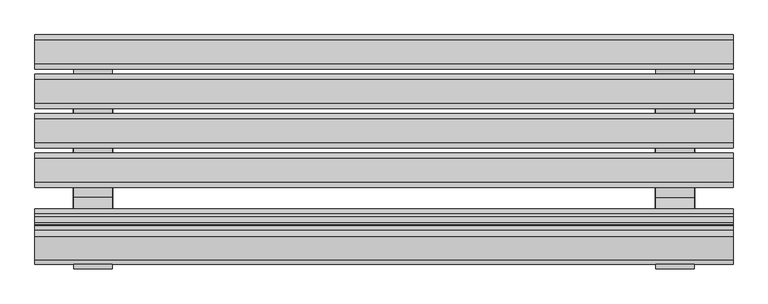
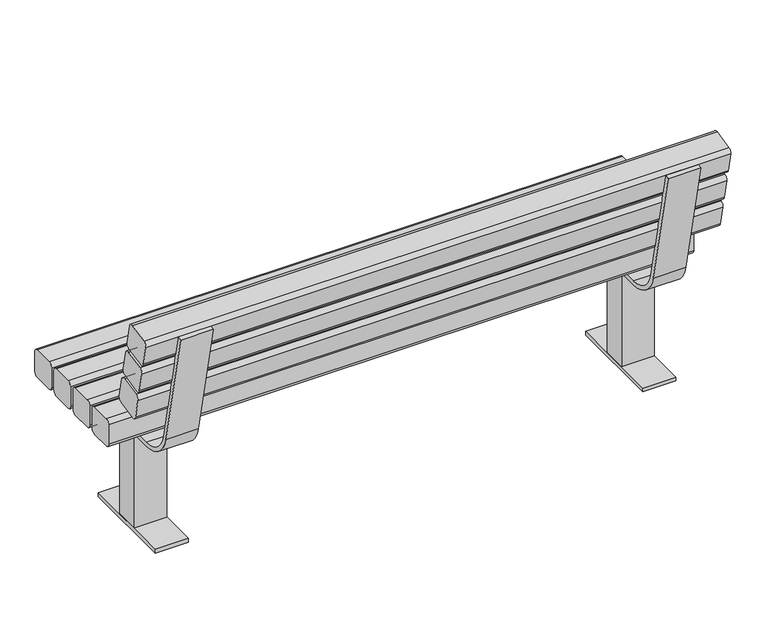
"""IFC4 building model written with IfcOpenShell, lengths in millimetres: furniture geometry, NLRS_90_FU_WPB_parkbank_gen_rsf : 1800mm breed."""

from ifc_helpers import new_model, si_unit, point, frame, frame_2d, origin, origin_with_axes, place, context, project, spatial, polyline, circle_curve, trimmed, segment, composite_curve, outline, extrude, source, transform, mapped, element, save


def furniture_d88922e8(model_context):
    return source(origin(), model_context, "Body", "SweptSolid", [
        extrude(outline(polyline([(-778.4316018, 207.3631555), (-778.4316018, 512.1631555), (-676.8316018, 512.1631555), (-676.8316018, 207.3631555), (-778.4316018, 207.3631555)])), origin_with_axes(), (0.0, 0.0, 1.0), 12.7),
        extrude(outline(polyline([(722.3683982, 321.6631555), (722.3683982, 397.8631555), (822.3683982, 397.8631555), (822.3683982, 321.6631555), (722.3683982, 321.6631555)])), frame((0.0, 0.0, 12.7), z_axis=(0.0, 0.0, 1.0), x_axis=(1.0, 0.0, 0.0)), (0.0, 0.0, 1.0), 304.8),
        extrude(outline(composite_curve([segment(polyline([(85.9429731, 777.6296037), (165.0207138, 405.5980841)]), True, "CONTINUOUS"), segment(trimmed(circle_curve(frame_2d((258.1892727, 425.4016727)), 95.25), [point((165.0207138, 405.5980841))], [point((258.1892727, 330.1516727))], True, "CARTESIAN"), True, "CONTINUOUS"), segment(polyline([(258.1892727, 330.1516727), (656.6612098, 330.1516727), (656.6612098, 317.5), (258.1790004, 317.5)]), True, "CONTINUOUS"), segment(trimmed(circle_curve(frame_2d((258.1790004, 425.45)), 107.95), [point((258.1790004, 317.5))], [point((152.5879669, 403.005933))], False, "CARTESIAN"), True, "CONTINUOUS"), segment(polyline([(152.5879669, 403.005933), (73.5204986, 774.9891252), (85.9429731, 777.6296037)]), True, "CONTINUOUS")], self_intersect=False)), frame((722.3683982, 0.0, 0.0), z_axis=(1.0, 0.0, 0.0), x_axis=(0.0, 1.0, 0.0)), (0.0, 0.0, 1.0), 100.0),
        extrude(outline(polyline([(-677.6316018, 321.6631555), (-777.6316018, 321.6631555), (-777.6316018, 397.8631555), (-677.6316018, 397.8631555), (-677.6316018, 321.6631555)])), frame((0.0, 0.0, 12.7), z_axis=(0.0, 0.0, 1.0), x_axis=(1.0, 0.0, 0.0)), (0.0, 0.0, 1.0), 304.8),
        extrude(outline(polyline([(823.1683982, 207.3631555), (721.5683982, 207.3631555), (721.5683982, 512.1631555), (823.1683982, 512.1631555), (823.1683982, 207.3631555)])), origin_with_axes(), (0.0, 0.0, 1.0), 12.7),
        extrude(outline(composite_curve([segment(trimmed(circle_curve(frame_2d((202.7254759, 594.7128821)), 12.7), [point((200.0849974, 607.1353566))], [point((215.1479504, 597.3533605))], False, "CARTESIAN"), True, "CONTINUOUS"), segment(polyline([(215.1479504, 597.3533605), (228.3503428, 535.2409879)]), True, "CONTINUOUS"), segment(trimmed(circle_curve(frame_2d((215.9278683, 532.6005094)), 12.7), [point((228.3503428, 535.2409879))], [point((218.5683467, 520.1780349))], False, "CARTESIAN"), True, "CONTINUOUS"), segment(polyline([(218.5683467, 520.1780349), (156.4559741, 506.9756425)]), True, "CONTINUOUS"), segment(trimmed(circle_curve(frame_2d((153.8154956, 519.398117)), 12.7), [point((156.4559741, 506.9756425))], [point((141.3930211, 516.7576386))], False, "CARTESIAN"), True, "CONTINUOUS"), segment(polyline([(141.3930211, 516.7576386), (128.1906287, 578.8700112)]), True, "CONTINUOUS"), segment(trimmed(circle_curve(frame_2d((140.6131032, 581.5104897)), 12.7), [point((128.1906287, 578.8700112))], [point((137.9726248, 593.9329642))], False, "CARTESIAN"), True, "CONTINUOUS"), segment(polyline([(137.9726248, 593.9329642), (200.0849974, 607.1353566)]), True, "CONTINUOUS")], self_intersect=False)), frame((-877.6316018, 0.0, 0.0), z_axis=(1.0, 0.0, 0.0), x_axis=(0.0, 1.0, 0.0)), (0.0, 0.0, 1.0), 1800.0),
        extrude(outline(composite_curve([segment(trimmed(circle_curve(frame_2d((181.6016481, 694.0926783)), 12.7), [point((178.9611696, 706.5151528))], [point((194.0241226, 696.7331568))], False, "CARTESIAN"), True, "CONTINUOUS"), segment(polyline([(194.0241226, 696.7331568), (207.226515, 634.6207841)]), True, "CONTINUOUS"), segment(trimmed(circle_curve(frame_2d((194.8040405, 631.9803056)), 12.7), [point((207.226515, 634.6207841))], [point((197.4445189, 619.5578311))], False, "CARTESIAN"), True, "CONTINUOUS"), segment(polyline([(197.4445189, 619.5578311), (135.3321463, 606.3554388)]), True, "CONTINUOUS"), segment(trimmed(circle_curve(frame_2d((132.6916678, 618.7779133)), 12.7), [point((135.3321463, 606.3554388))], [point((120.2691933, 616.1374348))], False, "CARTESIAN"), True, "CONTINUOUS"), segment(polyline([(120.2691933, 616.1374348), (107.0668009, 678.2498075)]), True, "CONTINUOUS"), segment(trimmed(circle_curve(frame_2d((119.4892755, 680.8902859)), 12.7), [point((107.0668009, 678.2498075))], [point((116.848797, 693.3127605))], False, "CARTESIAN"), True, "CONTINUOUS"), segment(polyline([(116.848797, 693.3127605), (178.9611696, 706.5151528)]), True, "CONTINUOUS")], self_intersect=False)), frame((-877.6316018, 0.0, 0.0), z_axis=(1.0, 0.0, 0.0), x_axis=(0.0, 1.0, 0.0)), (0.0, 0.0, 1.0), 1800.0),
        extrude(outline(composite_curve([segment(polyline([(85.9429731, 777.6296037), (165.0207138, 405.5980841)]), True, "CONTINUOUS"), segment(trimmed(circle_curve(frame_2d((258.1892727, 425.4016727)), 95.25), [point((165.0207138, 405.5980841))], [point((258.1892727, 330.1516727))], True, "CARTESIAN"), True, "CONTINUOUS"), segment(polyline([(258.1892727, 330.1516727), (656.6612098, 330.1516727), (656.6612098, 317.5), (258.1790004, 317.5)]), True, "CONTINUOUS"), segment(trimmed(circle_curve(frame_2d((258.1790004, 425.45)), 107.95), [point((258.1790004, 317.5))], [point((152.5879669, 403.005933))], False, "CARTESIAN"), True, "CONTINUOUS"), segment(polyline([(152.5879669, 403.005933), (73.5204986, 774.9891252), (85.9429731, 777.6296037)]), True, "CONTINUOUS")], self_intersect=False)), frame((-777.6316018, 0.0, 0.0), z_axis=(1.0, 0.0, 0.0), x_axis=(0.0, 1.0, 0.0)), (0.0, 0.0, 1.0), 100.0),
        extrude(outline(composite_curve([segment(trimmed(circle_curve(frame_2d((160.4778203, 793.4724745)), 12.7), [point((157.8373418, 805.8949491))], [point((172.9002948, 796.112953))], False, "CARTESIAN"), True, "CONTINUOUS"), segment(polyline([(172.9002948, 796.112953), (186.1026872, 734.0005804)]), True, "CONTINUOUS"), segment(trimmed(circle_curve(frame_2d((173.6802127, 731.3601019)), 12.7), [point((186.1026872, 734.0005804))], [point((176.3206912, 718.9376274))], False, "CARTESIAN"), True, "CONTINUOUS"), segment(polyline([(176.3206912, 718.9376274), (114.2083185, 705.735235)]), True, "CONTINUOUS"), segment(trimmed(circle_curve(frame_2d((111.56784, 718.1577095)), 12.7), [point((114.2083185, 705.735235))], [point((99.1453655, 715.517231))], False, "CARTESIAN"), True, "CONTINUOUS"), segment(polyline([(99.1453655, 715.517231), (85.9429731, 777.6296037)]), True, "CONTINUOUS"), segment(trimmed(circle_curve(frame_2d((98.3654477, 780.2700822)), 12.7), [point((85.9429731, 777.6296037))], [point((95.7249692, 792.6925567))], False, "CARTESIAN"), True, "CONTINUOUS"), segment(polyline([(95.7249692, 792.6925567), (157.8373418, 805.8949491)]), True, "CONTINUOUS")], self_intersect=False)), frame((-877.6316018, 0.0, 0.0), z_axis=(1.0, 0.0, 0.0), x_axis=(0.0, 1.0, 0.0)), (0.0, 0.0, 1.0), 1800.0),
        extrude(outline(composite_curve([segment(trimmed(circle_curve(frame_2d((665.0298429, 406.3516727)), 12.7), [point((665.0298429, 419.0516727))], [point((677.7298429, 406.3516727))], False, "CARTESIAN"), True, "CONTINUOUS"), segment(polyline([(677.7298429, 406.3516727), (677.7298429, 342.8516727)]), True, "CONTINUOUS"), segment(trimmed(circle_curve(frame_2d((665.0298429, 342.8516727)), 12.7), [point((677.7298429, 342.8516727))], [point((665.0298429, 330.1516727))], False, "CARTESIAN"), True, "CONTINUOUS"), segment(polyline([(665.0298429, 330.1516727), (601.5298429, 330.1516727)]), True, "CONTINUOUS"), segment(trimmed(circle_curve(frame_2d((601.5298429, 342.8516727)), 12.7), [point((601.5298429, 330.1516727))], [point((588.8298429, 342.8516727))], False, "CARTESIAN"), True, "CONTINUOUS"), segment(polyline([(588.8298429, 342.8516727), (588.8298429, 406.3516727)]), True, "CONTINUOUS"), segment(trimmed(circle_curve(frame_2d((601.5298429, 406.3516727)), 12.7), [point((588.8298429, 406.3516727))], [point((601.5298429, 419.0516727))], False, "CARTESIAN"), True, "CONTINUOUS"), segment(polyline([(601.5298429, 419.0516727), (665.0298429, 419.0516727)]), True, "CONTINUOUS")], self_intersect=False)), frame((-877.6316018, 0.0, 0.0), z_axis=(1.0, 0.0, 0.0), x_axis=(0.0, 1.0, 0.0)), (0.0, 0.0, 1.0), 1800.0),
        extrude(outline(composite_curve([segment(trimmed(circle_curve(frame_2d((563.4298429, 406.3516727)), 12.7), [point((563.4298429, 419.0516727))], [point((576.1298429, 406.3516727))], False, "CARTESIAN"), True, "CONTINUOUS"), segment(polyline([(576.1298429, 406.3516727), (576.1298429, 342.8516727)]), True, "CONTINUOUS"), segment(trimmed(circle_curve(frame_2d((563.4298429, 342.8516727)), 12.7), [point((576.1298429, 342.8516727))], [point((563.4298429, 330.1516727))], False, "CARTESIAN"), True, "CONTINUOUS"), segment(polyline([(563.4298429, 330.1516727), (499.9298429, 330.1516727)]), True, "CONTINUOUS"), segment(trimmed(circle_curve(frame_2d((499.9298429, 342.8516727)), 12.7), [point((499.9298429, 330.1516727))], [point((487.2298429, 342.8516727))], False, "CARTESIAN"), True, "CONTINUOUS"), segment(polyline([(487.2298429, 342.8516727), (487.2298429, 406.3516727)]), True, "CONTINUOUS"), segment(trimmed(circle_curve(frame_2d((499.9298429, 406.3516727)), 12.7), [point((487.2298429, 406.3516727))], [point((499.9298429, 419.0516727))], False, "CARTESIAN"), True, "CONTINUOUS"), segment(polyline([(499.9298429, 419.0516727), (563.4298429, 419.0516727)]), True, "CONTINUOUS")], self_intersect=False)), frame((-877.6316018, 0.0, 0.0), z_axis=(1.0, 0.0, 0.0), x_axis=(0.0, 1.0, 0.0)), (0.0, 0.0, 1.0), 1800.0),
        extrude(outline(composite_curve([segment(trimmed(circle_curve(frame_2d((461.8298429, 406.3516727)), 12.7), [point((461.8298429, 419.0516727))], [point((474.5298429, 406.3516727))], False, "CARTESIAN"), True, "CONTINUOUS"), segment(polyline([(474.5298429, 406.3516727), (474.5298429, 342.8516727)]), True, "CONTINUOUS"), segment(trimmed(circle_curve(frame_2d((461.8298429, 342.8516727)), 12.7), [point((474.5298429, 342.8516727))], [point((461.8298429, 330.1516727))], False, "CARTESIAN"), True, "CONTINUOUS"), segment(polyline([(461.8298429, 330.1516727), (398.3298429, 330.1516727)]), True, "CONTINUOUS"), segment(trimmed(circle_curve(frame_2d((398.3298429, 342.8516727)), 12.7), [point((398.3298429, 330.1516727))], [point((385.6298429, 342.8516727))], False, "CARTESIAN"), True, "CONTINUOUS"), segment(polyline([(385.6298429, 342.8516727), (385.6298429, 406.3516727)]), True, "CONTINUOUS"), segment(trimmed(circle_curve(frame_2d((398.3298429, 406.3516727)), 12.7), [point((385.6298429, 406.3516727))], [point((398.3298429, 419.0516727))], False, "CARTESIAN"), True, "CONTINUOUS"), segment(polyline([(398.3298429, 419.0516727), (461.8298429, 419.0516727)]), True, "CONTINUOUS")], self_intersect=False)), frame((-877.6316018, 0.0, 0.0), z_axis=(1.0, 0.0, 0.0), x_axis=(0.0, 1.0, 0.0)), (0.0, 0.0, 1.0), 1800.0),
        extrude(outline(composite_curve([segment(trimmed(circle_curve(frame_2d((360.2298429, 406.3516727)), 12.7), [point((360.2298429, 419.0516727))], [point((372.9298429, 406.3516727))], False, "CARTESIAN"), True, "CONTINUOUS"), segment(polyline([(372.9298429, 406.3516727), (372.9298429, 342.8516727)]), True, "CONTINUOUS"), segment(trimmed(circle_curve(frame_2d((360.2298429, 342.8516727)), 12.7), [point((372.9298429, 342.8516727))], [point((360.2298429, 330.1516727))], False, "CARTESIAN"), True, "CONTINUOUS"), segment(polyline([(360.2298429, 330.1516727), (296.7298429, 330.1516727)]), True, "CONTINUOUS"), segment(trimmed(circle_curve(frame_2d((296.7298429, 342.8516727)), 12.7), [point((296.7298429, 330.1516727))], [point((284.0298429, 342.8516727))], False, "CARTESIAN"), True, "CONTINUOUS"), segment(polyline([(284.0298429, 342.8516727), (284.0298429, 406.3516727)]), True, "CONTINUOUS"), segment(trimmed(circle_curve(frame_2d((296.7298429, 406.3516727)), 12.7), [point((284.0298429, 406.3516727))], [point((296.7298429, 419.0516727))], False, "CARTESIAN"), True, "CONTINUOUS"), segment(polyline([(296.7298429, 419.0516727), (360.2298429, 419.0516727)]), True, "CONTINUOUS")], self_intersect=False)), frame((-877.6316018, 0.0, 0.0), z_axis=(1.0, 0.0, 0.0), x_axis=(0.0, 1.0, 0.0)), (0.0, 0.0, 1.0), 1800.0),
    ])


if __name__ == "__main__":
    model = new_model("IFC4")
    model_context = context("Model", 3, world=origin())
    ifc_project = project(units=[si_unit("LENGTHUNIT", "METRE", prefix="MILLI")], contexts=[model_context])
    site = spatial("IfcSite", under=ifc_project)
    building = spatial("IfcBuilding", under=site)
    placement = place(None, origin())
    furniture_shape = furniture_d88922e8(model_context)
    element("IfcFurniture", 1, ObjectType="NLRS_90_FU_WPB_parkbank_gen_rsf : 1800mm breed", at=placement, inside=building, context=model_context, shape_type="MappedRepresentation", body=[
        mapped(furniture_shape, transform((0.0, 0.0, 0.0), x_axis=(1.0, 0.0, 0.0), y_axis=(0.0, 1.0, 0.0), z_axis=(0.0, 0.0, 1.0))),
    ])
    save(model, "model.ifc")

# Revit data of these elements
# Type "NLRS_90_FU_WPB_parkbank_gen_rsf : 1800mm breed"
#   Type IFC Predefined Type = "USERDEFINED"
#   Export Type to IFC As = "IfcGeographicElementType"
#   Type IfcGUID = "05J6pyYiTDtR2exmlhyPly"
#   IfcName[Type] = "parkbank 1800mm breed"
#   IfcDescription[Type] = "parkbank b 1800mm"
#   IfcObjectType[Type] = "BENCH"
#   IfcExportAs[Type] = "IfcGeographicElementType"
#   IfcExportType[Type] = "USERDEFINED"
#   NLRS_C_revit_versie = ""
#   NLRS_C_omschrijving_02 = "onderstel"
#   NLRS_C_omschrijving_01 = "zitting"
#   NLRS_C_content_versie = ""
#   NLRS_C_content_provider = ""
#   NLRS_C_content_handleiding = ""
#   NLRS_C_content_datum_uitgifte = ""
#   NLRS_C_content_datum_gewijzigd = ""
#   NLRS_C_content_creator = ""
#   Model = "generiek"
#   Manufacturer = "Revit Standards Foundation"
#   Description = "parkbank b 1800mm"
#   Assembly Code = "90.71"
#   bf_overstek = 150.00 mm
#   NLRS_C_hoogte_01 [instance default] = 419.052 mm
#   NLRS_C_hoogte [instance default] = 806.45 mm
#   NLRS_C_diepte_01 [instance default] = 372.631 mm
#   NLRS_C_breedte = 1800.00 mm
#   Default Elevation = 1219.20 mm
#   NLRS_C_materiaal_02 = NLRS_h2_staal mat gepolijst grijs_gen_rsf
#   NLRS_C_materiaal_01 = NLRS_i3_hout loofhout meranti vernis_gen_rsf
# Element 1 (IfcFurniture, "NLRS_90_FU_WPB_parkbank_gen_rsf : 1800mm breed")
#   Materials on its faces: "NLRS_i3_hout loofhout meranti vernis_gen_rsf", "NLRS_h2_staal mat gepolijst grijs_gen_rsf"
# Materials
#   "NLRS_h2_staal mat gepolijst grijs_gen_rsf": class "System", colour RGB 189 187 185, transparency 0, Keynote = "h2", Model = "generiek", Manufacturer = "Revit Standards Foundation", URL = "www.revitstandards.org", Description = "staal mat gepolijst", Cost = 0
#   "NLRS_i3_hout loofhout meranti vernis_gen_rsf": class "Unassigned", colour RGB 227 170 128, transparency 0, Keynote = "i3", Model = "generiek", Manufacturer = "Revit Standards Foundation", URL = "www.revitstandards.org", Description = "loofhout merantie vernis", Cost = 0
